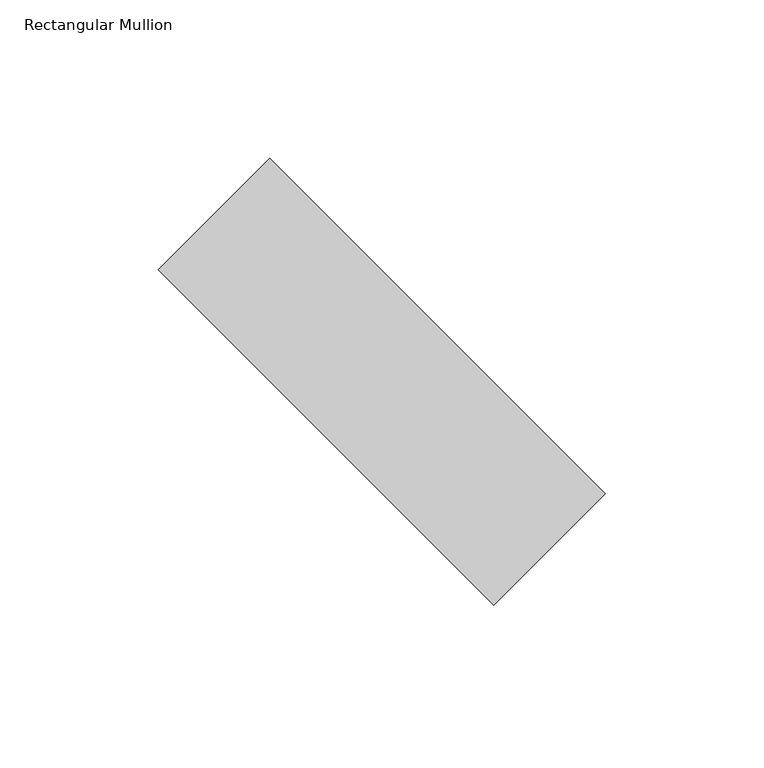
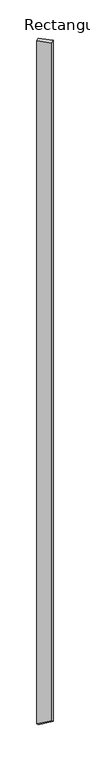
"""IFC4 building model written with IfcOpenShell, lengths in millimetres: member geometry, Rectangular Mullion : tilted mullions."""

from ifc_helpers import new_model, si_unit, origin, place, context, project, spatial, faceted_brep, source, transform, mapped, element, save


def rectangular_mullion_ddbb4f50(model_context):
    return source(origin(), model_context, "Body", "Brep", [
        faceted_brep([(-35.3553391, 70.7106781, 0.0), (-70.7106781, 35.3553391, 0.0), (35.3553391, -70.7106781, 0.0), (70.7106781, -35.3553391, 0.0), (-35.3553391, 70.7106781, -8054.2881412), (-70.7106781, 35.3553391, -8009.2546194), (35.3553391, -70.7106781, -7944.0791851), (70.7106781, -35.3553391, -7989.1127069)], [[[0, 1, 2, 3]], [[1, 0, 4, 5]], [[2, 1, 5, 6]], [[3, 2, 6, 7]], [[0, 3, 7, 4]], [[4, 7, 6, 5]]]),
    ])


if __name__ == "__main__":
    model = new_model("IFC4")
    model_context = context("Model", 3, world=origin())
    ifc_project = project(units=[si_unit("LENGTHUNIT", "METRE", prefix="MILLI")], contexts=[model_context])
    site = spatial("IfcSite", under=ifc_project)
    building = spatial("IfcBuilding", under=site)
    placement = place(None, origin())
    rectangular_mullion_shape = rectangular_mullion_ddbb4f50(model_context)
    element("IfcMember", 1, ObjectType="Rectangular Mullion : tilted mullions", at=placement, inside=building, context=model_context, shape_type="MappedRepresentation", body=[
        mapped(rectangular_mullion_shape, transform((0.0, 0.0, 0.0), x_axis=(1.0, 0.0, 0.0), y_axis=(0.0, 1.0, 0.0), z_axis=(0.0, 0.0, 1.0))),
    ])
    save(model, "model.ifc")

# Revit data of these elements
# Type "Rectangular Mullion : tilted mullions"
#   built-in parameter 1007304 = 0.492126 (stored number, unit not read)
#   built-in parameter 1007301 = 0.082021 (stored number, unit not read)
#   built-in parameter 1007300 = 0.082021 (stored number, unit not read)
# Element 1 (IfcMember, "Rectangular Mullion : tilted mullions")
#   Materials on its faces: "Aluminum"
# Materials
#   "Aluminum": class "Metal", colour RGB 244 244 244, transparency 0, Description = "Aluminum 6061", Cost = 0
